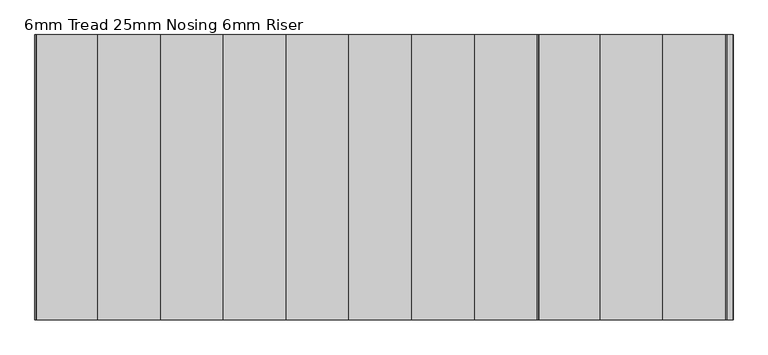
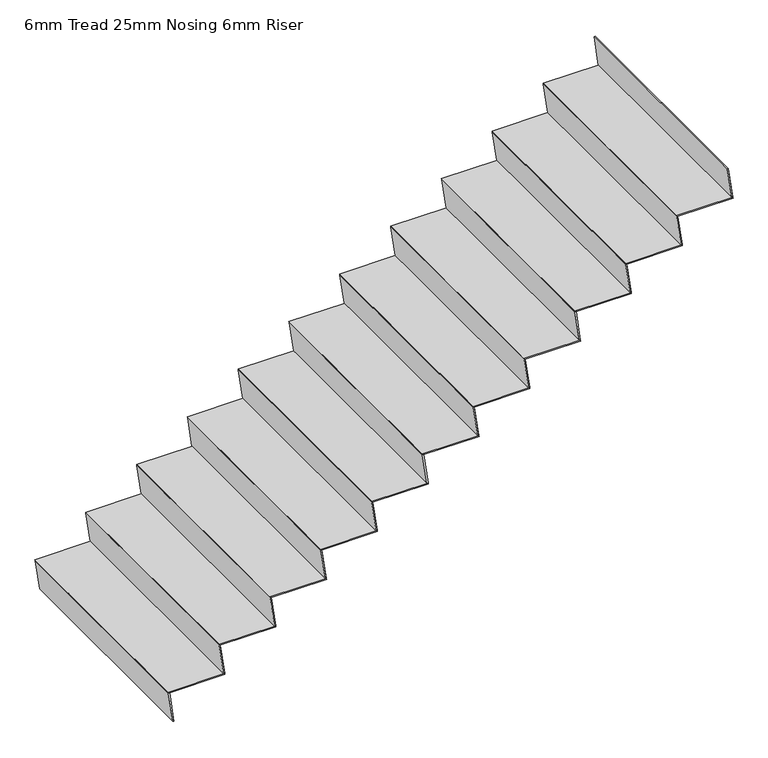
"""IFC4 building model written with IfcOpenShell, lengths in millimetres: stair flight geometry, 6mm Tread 25mm Nosing 6mm Riser."""

from ifc_helpers import new_model, si_unit, frame, origin, place, context, project, spatial, polyline, outline, extrude, source, transform, mapped, element, save


def stair_flight_6mm_tread_25mm_nosing_6mm_riser_0f826342(model_context):
    return source(origin(), model_context, "Body", "SweptSolid", [
        extrude(outline(polyline([(16470.5882353, 13631.0599092), (16470.5882353, 13325.0), (16464.5882353, 13325.85), (16464.5882353, 13631.9099092), (16470.5882353, 13631.0599092)])), frame((0.0, 10220.4345331, 0.0), z_axis=(0.0, 1.0, 0.0), x_axis=(0.0, 0.0, 1.0)), (0.0, 0.0, 1.0), 1250.0),
        extrude(outline(polyline([(16464.5882353, 13325.85), (16294.1176471, 13350.0), (16294.1176471, 13356.0599092), (16464.5882353, 13331.9099092), (16464.5882353, 13325.85)])), frame((0.0, 10220.4345331, 0.0), z_axis=(0.0, 1.0, 0.0), x_axis=(0.0, 0.0, 1.0)), (0.0, 0.0, 1.0), 1250.0),
        extrude(outline(polyline([(16641.0588235, 13600.85), (16470.5882353, 13625.0), (16470.5882353, 13631.0599092), (16641.0588235, 13606.9099092), (16641.0588235, 13600.85)])), frame((0.0, 10220.4345331, 0.0), z_axis=(0.0, 1.0, 0.0), x_axis=(0.0, 0.0, 1.0)), (0.0, 0.0, 1.0), 1250.0),
        extrude(outline(polyline([(16647.0588235, 13906.0599092), (16647.0588235, 13600.0), (16641.0588235, 13600.85), (16641.0588235, 13906.9099092), (16647.0588235, 13906.0599092)])), frame((0.0, 10220.4345331, 0.0), z_axis=(0.0, 1.0, 0.0), x_axis=(0.0, 0.0, 1.0)), (0.0, 0.0, 1.0), 1250.0),
        extrude(outline(polyline([(16817.5294118, 13875.85), (16647.0588235, 13900.0), (16647.0588235, 13906.0599092), (16817.5294118, 13881.9099092), (16817.5294118, 13875.85)])), frame((0.0, 10220.4345331, 0.0), z_axis=(0.0, 1.0, 0.0), x_axis=(0.0, 0.0, 1.0)), (0.0, 0.0, 1.0), 1250.0),
        extrude(outline(polyline([(16823.5294118, 14181.0599092), (16823.5294118, 13875.0), (16817.5294118, 13875.85), (16817.5294118, 14181.9099092), (16823.5294118, 14181.0599092)])), frame((0.0, 10220.4345331, 0.0), z_axis=(0.0, 1.0, 0.0), x_axis=(0.0, 0.0, 1.0)), (0.0, 0.0, 1.0), 1250.0),
        extrude(outline(polyline([(16994.0, 14150.85), (16823.5294118, 14175.0), (16823.5294118, 14181.0599092), (16994.0, 14156.9099092), (16994.0, 14150.85)])), frame((0.0, 10220.4345331, 0.0), z_axis=(0.0, 1.0, 0.0), x_axis=(0.0, 0.0, 1.0)), (0.0, 0.0, 1.0), 1250.0),
        extrude(outline(polyline([(17000.0, 14456.0599092), (17000.0, 14150.0), (16994.0, 14150.85), (16994.0, 14456.9099092), (17000.0, 14456.0599092)])), frame((0.0, 10220.4345331, 0.0), z_axis=(0.0, 1.0, 0.0), x_axis=(0.0, 0.0, 1.0)), (0.0, 0.0, 1.0), 1250.0),
        extrude(outline(polyline([(17170.4705882, 14425.85), (17000.0, 14450.0), (17000.0, 14456.0599092), (17170.4705882, 14431.9099092), (17170.4705882, 14425.85)])), frame((0.0, 10220.4345331, 0.0), z_axis=(0.0, 1.0, 0.0), x_axis=(0.0, 0.0, 1.0)), (0.0, 0.0, 1.0), 1250.0),
        extrude(outline(polyline([(17176.4705882, 14731.0599092), (17176.4705882, 14425.0), (17170.4705882, 14425.85), (17170.4705882, 14731.9099092), (17176.4705882, 14731.0599092)])), frame((0.0, 10220.4345331, 0.0), z_axis=(0.0, 1.0, 0.0), x_axis=(0.0, 0.0, 1.0)), (0.0, 0.0, 1.0), 1250.0),
        extrude(outline(polyline([(17346.9411765, 14700.85), (17176.4705882, 14725.0), (17176.4705882, 14731.0599092), (17346.9411765, 14706.9099092), (17346.9411765, 14700.85)])), frame((0.0, 10220.4345331, 0.0), z_axis=(0.0, 1.0, 0.0), x_axis=(0.0, 0.0, 1.0)), (0.0, 0.0, 1.0), 1250.0),
        extrude(outline(polyline([(17352.9411765, 15006.0599092), (17352.9411765, 14700.0), (17346.9411765, 14700.85), (17346.9411765, 15006.9099092), (17352.9411765, 15006.0599092)])), frame((0.0, 10220.4345331, 0.0), z_axis=(0.0, 1.0, 0.0), x_axis=(0.0, 0.0, 1.0)), (0.0, 0.0, 1.0), 1250.0),
        extrude(outline(polyline([(17523.4117647, 14975.85), (17352.9411765, 15000.0), (17352.9411765, 15006.0599092), (17523.4117647, 14981.9099092), (17523.4117647, 14975.85)])), frame((0.0, 10220.4345331, 0.0), z_axis=(0.0, 1.0, 0.0), x_axis=(0.0, 0.0, 1.0)), (0.0, 0.0, 1.0), 1250.0),
        extrude(outline(polyline([(17529.4117647, 15281.0599092), (17529.4117647, 14975.0), (17523.4117647, 14975.85), (17523.4117647, 15281.9099092), (17529.4117647, 15281.0599092)])), frame((0.0, 10220.4345331, 0.0), z_axis=(0.0, 1.0, 0.0), x_axis=(0.0, 0.0, 1.0)), (0.0, 0.0, 1.0), 1250.0),
        extrude(outline(polyline([(17699.8823529, 15250.85), (17529.4117647, 15275.0), (17529.4117647, 15281.0599092), (17699.8823529, 15256.9099092), (17699.8823529, 15250.85)])), frame((0.0, 10220.4345331, 0.0), z_axis=(0.0, 1.0, 0.0), x_axis=(0.0, 0.0, 1.0)), (0.0, 0.0, 1.0), 1250.0),
        extrude(outline(polyline([(17705.8823529, 15556.0599092), (17705.8823529, 15250.0), (17699.8823529, 15250.85), (17699.8823529, 15556.9099092), (17705.8823529, 15556.0599092)])), frame((0.0, 10220.4345331, 0.0), z_axis=(0.0, 1.0, 0.0), x_axis=(0.0, 0.0, 1.0)), (0.0, 0.0, 1.0), 1250.0),
        extrude(outline(polyline([(17876.3529412, 15525.85), (17705.8823529, 15550.0), (17705.8823529, 15556.0599092), (17876.3529412, 15531.9099092), (17876.3529412, 15525.85)])), frame((0.0, 10220.4345331, 0.0), z_axis=(0.0, 1.0, 0.0), x_axis=(0.0, 0.0, 1.0)), (0.0, 0.0, 1.0), 1250.0),
        extrude(outline(polyline([(17882.3529412, 15831.0599092), (17882.3529412, 15525.0), (17876.3529412, 15525.85), (17876.3529412, 15831.9099092), (17882.3529412, 15831.0599092)])), frame((0.0, 10220.4345331, 0.0), z_axis=(0.0, 1.0, 0.0), x_axis=(0.0, 0.0, 1.0)), (0.0, 0.0, 1.0), 1250.0),
        extrude(outline(polyline([(18052.8235294, 15800.85), (17882.3529412, 15825.0), (17882.3529412, 15831.0599092), (18052.8235294, 15806.9099092), (18052.8235294, 15800.85)])), frame((0.0, 10220.4345331, 0.0), z_axis=(0.0, 1.0, 0.0), x_axis=(0.0, 0.0, 1.0)), (0.0, 0.0, 1.0), 1250.0),
        extrude(outline(polyline([(18058.8235294, 16106.0599092), (18058.8235294, 15800.0), (18052.8235294, 15800.85), (18052.8235294, 16106.9099092), (18058.8235294, 16106.0599092)])), frame((0.0, 10220.4345331, 0.0), z_axis=(0.0, 1.0, 0.0), x_axis=(0.0, 0.0, 1.0)), (0.0, 0.0, 1.0), 1250.0),
        extrude(outline(polyline([(18229.2941176, 16075.85), (18058.8235294, 16100.0), (18058.8235294, 16106.0599092), (18229.2941176, 16081.9099092), (18229.2941176, 16075.85)])), frame((0.0, 10220.4345331, 0.0), z_axis=(0.0, 1.0, 0.0), x_axis=(0.0, 0.0, 1.0)), (0.0, 0.0, 1.0), 1250.0),
        extrude(outline(polyline([(18405.7647059, 16350.85), (18235.2941176, 16375.0), (18235.2941176, 16381.0599092), (18405.7647059, 16356.9099092), (18405.7647059, 16350.85)])), frame((0.0, 10220.4345331, 0.0), z_axis=(0.0, 1.0, 0.0), x_axis=(0.0, 0.0, 1.0)), (0.0, 0.0, 1.0), 1250.0),
        extrude(outline(polyline([(18235.2941176, 16381.0599092), (18235.2941176, 16075.0), (18229.2941176, 16075.85), (18229.2941176, 16381.9099092), (18235.2941176, 16381.0599092)])), frame((0.0, 10220.4345331, 0.0), z_axis=(0.0, 1.0, 0.0), x_axis=(0.0, 0.0, 1.0)), (0.0, 0.0, 1.0), 1250.0),
    ])


if __name__ == "__main__":
    model = new_model("IFC4")
    model_context = context("Model", 3, world=origin())
    ifc_project = project(units=[si_unit("LENGTHUNIT", "METRE", prefix="MILLI")], contexts=[model_context])
    site = spatial("IfcSite", under=ifc_project)
    building = spatial("IfcBuilding", under=site)
    placement = place(None, origin())
    stair_flight_6mm_tread_25mm_nosing_6mm_riser_shape = stair_flight_6mm_tread_25mm_nosing_6mm_riser_0f826342(model_context)
    element("IfcStairFlight", 1, ObjectType="6mm Tread 25mm Nosing 6mm Riser", at=placement, inside=building, context=model_context, shape_type="MappedRepresentation", body=[
        mapped(stair_flight_6mm_tread_25mm_nosing_6mm_riser_shape, transform((0.0, 0.0, 0.0), x_axis=(1.0, 0.0, 0.0), y_axis=(0.0, 1.0, 0.0), z_axis=(0.0, 0.0, 1.0))),
    ])
    save(model, "model.ifc")

# Revit data of these elements
# Element 1 (IfcStairFlight, "6mm Tread 25mm Nosing 6mm Riser")
#   Materials on its faces: "Steel, Paint Finish, Dark Gray"
# Materials
#   "Steel, Paint Finish, Dark Gray": class "Metal", colour RGB 89 89 89, transparency 0, Description = "Steel, paint finish, dark gray, glossy", Cost = 0
